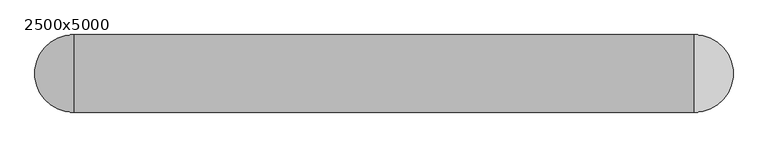
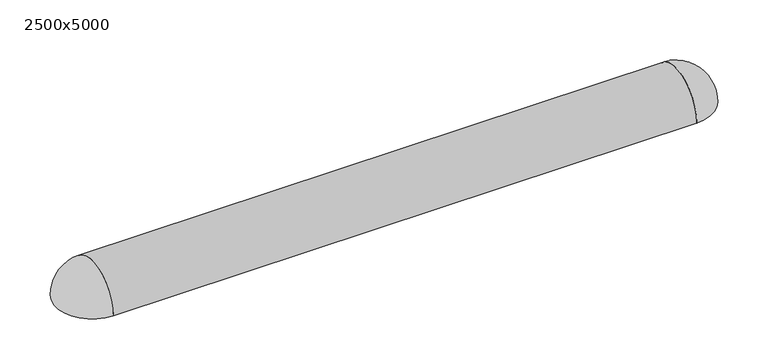
"""IFC4 building model written with IfcOpenShell, lengths in millimetres: proxy geometry, NLRS_71_PA_LB_parkeer-vak-recht_gen_rsf : 2500x5000."""

from ifc_helpers import new_model, si_unit, point, frame, frame_2d, origin, place, context, project, spatial, polyline, circle_curve, ellipse_curve, trimmed, segment, composite_curve, outline, extrude, source, transform, mapped, element, save
from ifc_brep_helpers import plane_surface, revolved_surface, advanced_brep


def proxy_2500x5000_b4be1f3b(model_context):
    return source(origin(), model_context, "Body", "SolidModel", [
        advanced_brep(
        [(-800.0, -1749.9000123, 0.0), (-800.0, -1949.9000123, 0.0)],
        [
            (0, 1),
            (1, 0, circle_curve(frame((-800.0, -1849.9000123, 0.0), z_axis=(0.0, 0.0, -1.0), x_axis=(0.0, 1.0, 0.0)), 100.0)),
            (0, 1, circle_curve(frame((-800.0, -1849.9000123, 0.0), z_axis=(1.0, 0.0, 0.0), x_axis=(0.0, 1.0, 0.0)), 100.0)),
        ],
        [
            plane_surface(frame((-800.0, -1534.9000123, 0.0), z_axis=(0.0, 0.0, -1.0), x_axis=(-1.0, 0.0, 0.0))),
            plane_surface(frame((-800.0, -1534.9000123, 0.0), z_axis=(1.0, 0.0, 0.0), x_axis=(0.0, 0.0, 1.0))),
            revolved_surface(trimmed(ellipse_curve(frame((-800.0, -1849.9000123, 0.0), z_axis=(0.0, 0.0, -1.0), x_axis=(0.0, 1.0, 0.0)), 100.0, 100.0), [point((-800.0, -1949.9000123, 0.0))], [point((-800.0, -1749.9000123, 0.0))], True, "CARTESIAN"), (-800.0, -1534.9000123, 0.0), (0.0, 1.0, 0.0)),
        ],
        [
            (0, [[1, 2]]),
            (1, [[-1, 3]]),
            (2, [[-3, -2]]),
        ],
    ),
        advanced_brep(
        [(800.0, -1749.9000123, 0.0), (800.0, -1949.9000123, 0.0)],
        [
            (0, 1, circle_curve(frame((800.0, -1849.9000123, 0.0), z_axis=(0.0, 0.0, -1.0), x_axis=(0.0, 1.0, 0.0)), 100.0)),
            (1, 0),
            (1, 0, circle_curve(frame((800.0, -1849.9000123, 0.0), z_axis=(-1.0, 0.0, 0.0), x_axis=(0.0, 1.0, 0.0)), 100.0)),
        ],
        [
            plane_surface(frame((800.0, -1534.9000123, 0.0), z_axis=(0.0, 0.0, -1.0), x_axis=(1.0, 0.0, 0.0))),
            plane_surface(frame((800.0, -1534.9000123, 0.0), z_axis=(-1.0, 0.0, 0.0), x_axis=(0.0, 0.0, 1.0))),
            revolved_surface(trimmed(ellipse_curve(frame((800.0, -1849.9000123, 0.0), z_axis=(0.0, 0.0, -1.0), x_axis=(0.0, 1.0, 0.0)), 100.0, 100.0), [point((800.0, -1749.9000123, 0.0))], [point((800.0, -1949.9000123, 0.0))], True, "CARTESIAN"), (800.0, -1534.9000123, 0.0), (0.0, -1.0, 0.0)),
        ],
        [
            (0, [[1, 2]]),
            (1, [[-2, 3]]),
            (2, [[-3, -1]]),
        ],
    ),
        extrude(outline(composite_curve([segment(trimmed(circle_curve(frame_2d((-1849.9000123, 0.0)), 100.0), [point((-1949.9000123, 0.0))], [point((-1749.9000123, 0.0))], False, "CARTESIAN"), True, "CONTINUOUS"), segment(polyline([(-1749.9000123, 0.0), (-1949.9000123, 0.0)]), True, "CONTINUOUS")], self_intersect=False)), frame((-800.0, 0.0, 0.0), z_axis=(1.0, 0.0, 0.0), x_axis=(0.0, 1.0, 0.0)), (0.0, 0.0, 1.0), 1600.0),
    ])


if __name__ == "__main__":
    model = new_model("IFC4")
    model_context = context("Model", 3, world=origin())
    ifc_project = project(units=[si_unit("LENGTHUNIT", "METRE", prefix="MILLI")], contexts=[model_context])
    site = spatial("IfcSite", under=ifc_project)
    building = spatial("IfcBuilding", under=site)
    placement = place(None, origin())
    proxy_2500x5000_shape = proxy_2500x5000_b4be1f3b(model_context)
    element("IfcBuildingElementProxy", 1, Name="NLRS_71_PA_LB_parkeer-vak-recht_gen_rsf : 2500x5000", ObjectType="NLRS_71_PA_LB_parkeer-vak-recht_gen_rsf : 2500x5000", at=placement, inside=building, context=model_context, shape_type="MappedRepresentation", body=[
        mapped(proxy_2500x5000_shape, transform((0.0, 0.0, 0.0), x_axis=(1.0, 0.0, 0.0), y_axis=(0.0, 1.0, 0.0), z_axis=(0.0, 0.0, 1.0))),
    ])
    save(model, "model.ifc")

# Revit data of these elements
# Type "NLRS_71_PA_LB_parkeer-vak-recht_gen_rsf : 2500x5000"
#   Type IFC Predefined Type = "USERDEFINED"
#   Export Type to IFC As = "IfcBuildingElementProxyType"
#   Type IfcGUID = "2C9lkgojj1sel6c4s_vTQW"
#   Description = "parkeervak recht bxd 2500x5000mm"
#   IfcName[Type] = "parkeervak 2500x5000"
#   IfcDescription[Type] = "parkeervak recht bxd 2500x5000mm"
#   IfcObjectType[Type] = "PARKINGSPACE"
#   IfcExportAs[Type] = "IfcBuildingElementProxyType"
#   IfcExportType[Type] = "USERDEFINED"
#   Assembly Code = "71.10"
#   NLRS_C_lengte = 5000.00 mm
#   NLRS_C_breedte = 2500.00 mm
#   rijbaan-6500 = no
#   rijbaan-5000 = yes
#   biggenrug B [instance default] = yes
#   biggenrug A [instance default] = yes
#   Electra aansluiting = no
#   Miva = no
#   materiaal_biggenrug = NLRS_f2_beton prefab_gen_rsf
# Element 1 (IfcBuildingElementProxy, "NLRS_71_PA_LB_parkeer-vak-recht_gen_rsf : 2500x5000")
#   Materials on its faces: "NLRS_f2_beton prefab_gen_rsf"
# Materials
#   "NLRS_f2_beton prefab_gen_rsf": class "F - Niet gebakken kunststeen", colour RGB 129 133 118, transparency 0, Keynote = "f2", Model = "generiek", Manufacturer = "Revit Standards Foundation", URL = "www.revitstandards.org", Description = "beton prefab", Cost = 0
